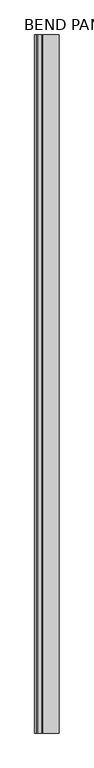
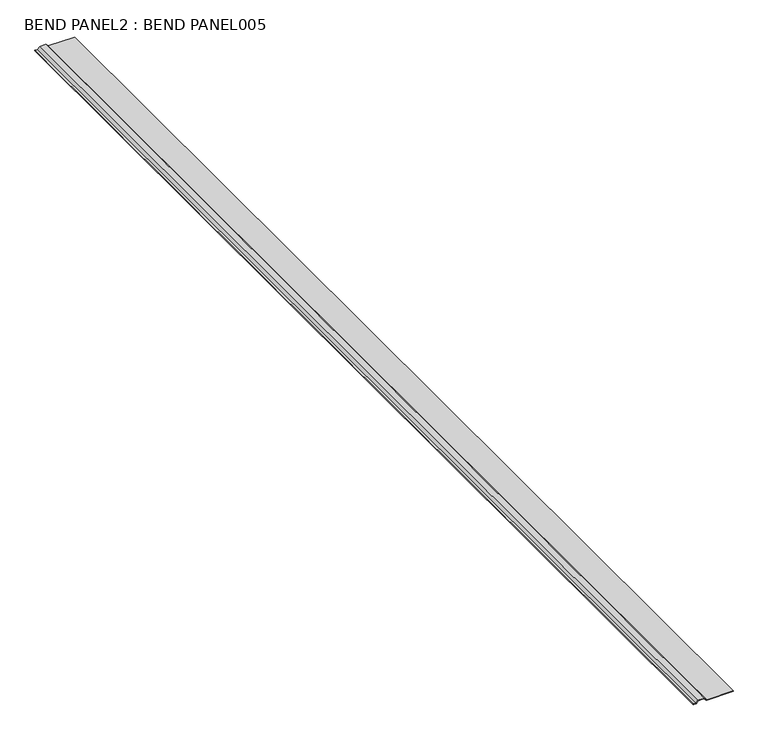
"""IFC4 building model written with IfcOpenShell, lengths in millimetres: proxy geometry, BEND PANEL2 : BEND PANEL005."""

from ifc_helpers import new_model, si_unit, point, frame, frame_2d, origin, place, context, project, spatial, polyline, circle_curve, trimmed, segment, composite_curve, outline, extrude, source, transform, mapped, element, save


def bend_panel2_bend_panel005_8c87a596(model_context):
    return source(origin(), model_context, "Body", "SweptSolid", [
        extrude(outline(composite_curve([segment(polyline([(42575.4212949, 5895.2230694), (42576.6119199, 5895.2230694), (42576.6119199, 5848.7155886), (42580.7948046, 5844.5327039), (42580.7948046, 5833.5642507), (42576.6119199, 5829.381366), (42576.6119199, 5825.5083246), (42575.4212949, 5825.5083246), (42575.4212949, 5829.381366)]), True, "CONTINUOUS"), segment(trimmed(circle_curve(frame_2d((42576.6119199, 5829.381366)), 1.190625), [point((42575.4212949, 5829.381366))], [point((42575.7700209, 5830.223265))], False, "CARTESIAN"), True, "CONTINUOUS"), segment(polyline([(42575.7700209, 5830.223265), (42579.6041796, 5834.0574237), (42579.6041796, 5844.0395308), (42575.7700209, 5847.8736895)]), True, "CONTINUOUS"), segment(trimmed(circle_curve(frame_2d((42576.6119199, 5848.7155885)), 1.190625), [point((42575.7700209, 5847.8736895))], [point((42575.4212949, 5848.7155885))], False, "CARTESIAN"), True, "CONTINUOUS"), segment(polyline([(42575.4212949, 5848.7155885), (42575.4212949, 5895.2230694)]), True, "CONTINUOUS")], self_intersect=False)), frame((0.0, -1052.8906574, 0.0), z_axis=(0.0, 1.0, 0.0), x_axis=(0.0, 0.0, 1.0)), (0.0, 0.0, 1.0), 1999.85),
    ])


if __name__ == "__main__":
    model = new_model("IFC4")
    model_context = context("Model", 3, world=origin())
    ifc_project = project(units=[si_unit("LENGTHUNIT", "METRE", prefix="MILLI")], contexts=[model_context])
    site = spatial("IfcSite", under=ifc_project)
    building = spatial("IfcBuilding", under=site)
    placement = place(None, origin())
    bend_panel2_bend_panel005_shape = bend_panel2_bend_panel005_8c87a596(model_context)
    element("IfcBuildingElementProxy", 1, Name="BEND PANEL2 : BEND PANEL005", ObjectType="BEND PANEL2 : BEND PANEL005", at=placement, inside=building, context=model_context, shape_type="MappedRepresentation", body=[
        mapped(bend_panel2_bend_panel005_shape, transform((0.0, 0.0, 0.0), x_axis=(1.0, 0.0, 0.0), y_axis=(0.0, 1.0, 0.0), z_axis=(0.0, 0.0, 1.0))),
    ])
    save(model, "model.ifc")

# Revit data of these elements
# Type "BEND PANEL2 : BEND PANEL005"
#   NameOverride = "BEND PANEL005"
# Element 1 (IfcBuildingElementProxy, "BEND PANEL2 : BEND PANEL005")
#   Materials on its faces: "METAL PROFILE"
# Materials
#   "METAL PROFILE": class "Unassigned", colour RGB 128 128 128, transparency 0
